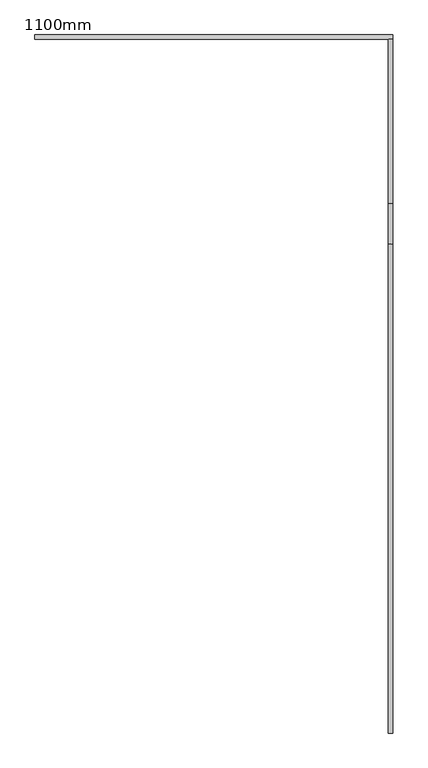
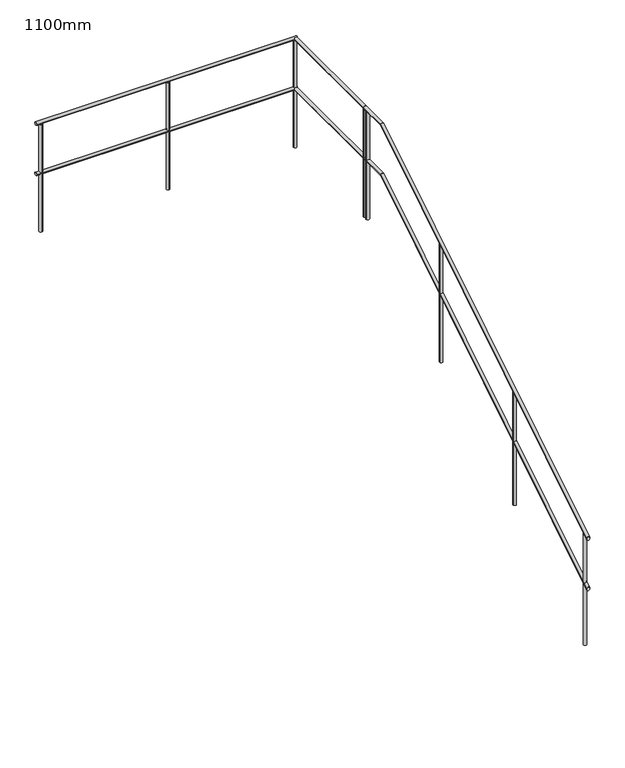
"""IFC4 building model written with IfcOpenShell, lengths in millimetres: railing geometry, 1100mm."""

from ifc_helpers import new_model, si_unit, point, frame, frame_2d, origin, place, context, project, spatial, circle_curve, ellipse_curve, trimmed, segment, composite_curve, outline, extrude, source, transform, mapped, element, save
from ifc_brep_helpers import plane_surface, cylinder_surface, advanced_brep


def railing_1100mm_f57b0715(model_context):
    return source(origin(), model_context, "Body", "SolidModel", [
        advanced_brep(
        [(12685.1052251, 14699.5208589, 456.3396197), (12655.1052251, 14699.5208589, 456.3396197), (12685.1052251, 18339.5208589, 2547.0), (12655.1052251, 18339.5208589, 2547.0), (12685.1052251, 18063.8019306, 2547.0), (12655.1052251, 18063.8019306, 2547.0)],
        [
            (0, 1, ellipse_curve(frame((12670.1052251, 14699.5208589, 456.3396197), z_axis=(0.0, -1.0, 0.0), x_axis=(0.0, 0.0, -1.0)), 17.6603803, 15.0)),
            (1, 0, ellipse_curve(frame((12670.1052251, 14699.5208589, 456.3396197), z_axis=(0.0, -1.0, 0.0), x_axis=(0.0, 0.0, -1.0)), 17.6603803, 15.0)),
            (2, 3, circle_curve(frame((12670.1052251, 18339.5208589, 2547.0), z_axis=(0.0, 1.0, 0.0), x_axis=(-1.0, 0.0, 0.0)), 15.0)),
            (3, 2, circle_curve(frame((12670.1052251, 18339.5208589, 2547.0), z_axis=(0.0, 1.0, 0.0), x_axis=(-1.0, 0.0, 0.0)), 15.0)),
            (0, 4),
            (4, 5, ellipse_curve(frame((12670.1052251, 18063.8019306, 2547.0), z_axis=(0.0, -0.9616025257983003, -0.2744459552959912), x_axis=(0.0, 0.2744459552959914, -0.9616025257983002)), 15.5989607, 15.0)),
            (5, 1),
            (5, 4, ellipse_curve(frame((12670.1052251, 18063.8019306, 2547.0), z_axis=(0.0, -0.9616025257983003, -0.2744459552959912), x_axis=(0.0, 0.2744459552959914, -0.9616025257983002)), 15.5989607, 15.0)),
            (4, 2),
            (3, 5),
        ],
        [
            plane_surface(frame((12670.1052251, 14699.5208589, 474.0), z_axis=(0.0, -1.0, 0.0), x_axis=(0.0, 0.0, 1.0))),
            plane_surface(frame((12670.1052251, 18339.5208589, 2562.0), z_axis=(0.0, 1.0, 0.0), x_axis=(0.0, 0.0, 1.0))),
            cylinder_surface(frame((12670.1052251, 14707.4380966, 461.2596175), z_axis=(0.0, -0.8493588352433417, -0.5278158476155052), x_axis=(-1.0, 0.0, 0.0)), 15.0),
            cylinder_surface(frame((12670.1052251, 18059.5208589, 2547.0), z_axis=(0.0, -1.0, 0.0), x_axis=(-1.0, 0.0, 0.0)), 15.0),
        ],
        [
            (0, [[1, 2]]),
            (1, [[3, 4]]),
            (2, [[-1, 5, 6, 7]]),
            (2, [[-2, -7, 8, -5]]),
            (3, [[-6, 9, -4, 10]]),
            (3, [[-8, -10, -3, -9]]),
        ],
    ),
        advanced_brep(
        [(12685.1052251, 18339.5208589, 2547.0), (12655.1052251, 18339.5208589, 2547.0), (12685.1052251, 19469.5208589, 2547.0), (12655.1052251, 19469.5208589, 2547.0)],
        [
            (0, 1, circle_curve(frame((12670.1052251, 18339.5208589, 2547.0), z_axis=(0.0, -1.0, 0.0), x_axis=(-1.0, 0.0, 0.0)), 15.0)),
            (1, 0, circle_curve(frame((12670.1052251, 18339.5208589, 2547.0), z_axis=(0.0, -1.0, 0.0), x_axis=(-1.0, 0.0, 0.0)), 15.0)),
            (2, 3, circle_curve(frame((12670.1052251, 19469.5208589, 2547.0), z_axis=(0.0, 1.0, 0.0), x_axis=(-1.0, 0.0, 0.0)), 15.0)),
            (3, 2, circle_curve(frame((12670.1052251, 19469.5208589, 2547.0), z_axis=(0.0, 1.0, 0.0), x_axis=(-1.0, 0.0, 0.0)), 15.0)),
            (0, 2),
            (3, 1),
        ],
        [
            plane_surface(frame((12670.1052251, 18339.5208589, 2562.0), z_axis=(0.0, -1.0, 0.0), x_axis=(0.0, 0.0, 1.0))),
            plane_surface(frame((12670.1052251, 19469.5208589, 2562.0), z_axis=(0.0, 1.0, 0.0), x_axis=(0.0, 0.0, 1.0))),
            cylinder_surface(frame((12670.1052251, 18339.5208589, 2547.0), z_axis=(0.0, -1.0, 0.0), x_axis=(-1.0, 0.0, 0.0)), 15.0),
        ],
        [
            (0, [[1, 2]]),
            (1, [[3, 4]]),
            (2, [[-1, 5, -4, 6]]),
            (2, [[-2, -6, -3, -5]]),
        ],
    ),
        advanced_brep(
        [(12685.1052251, 19499.5208589, 2547.0), (12685.1052251, 19469.5208589, 2547.0), (10225.1052251, 19499.5208589, 2547.0), (10225.1052251, 19469.5208589, 2547.0)],
        [
            (0, 1, circle_curve(frame((12685.1052251, 19484.5208589, 2547.0), z_axis=(1.0, 0.0, 0.0), x_axis=(0.0, -1.0, 0.0)), 15.0)),
            (1, 0, circle_curve(frame((12685.1052251, 19484.5208589, 2547.0), z_axis=(1.0, 0.0, 0.0), x_axis=(0.0, -1.0, 0.0)), 15.0)),
            (2, 3, circle_curve(frame((10225.1052251, 19484.5208589, 2547.0), z_axis=(-1.0, 0.0, 0.0), x_axis=(0.0, -1.0, 0.0)), 15.0)),
            (3, 2, circle_curve(frame((10225.1052251, 19484.5208589, 2547.0), z_axis=(-1.0, 0.0, 0.0), x_axis=(0.0, -1.0, 0.0)), 15.0)),
            (0, 2),
            (3, 1),
        ],
        [
            plane_surface(frame((12685.1052251, 19484.5208589, 2562.0), z_axis=(1.0, 0.0, 0.0), x_axis=(0.0, -1.0, 0.0))),
            plane_surface(frame((10225.1052251, 19484.5208589, 2562.0), z_axis=(-1.0, 0.0, 0.0), x_axis=(0.0, -1.0, 0.0))),
            cylinder_surface(frame((12685.1052251, 19484.5208589, 2547.0), z_axis=(1.0, 0.0, 0.0), x_axis=(0.0, -1.0, 0.0)), 15.0),
        ],
        [
            (0, [[1, 2]]),
            (1, [[3, 4]]),
            (2, [[-1, 5, -4, 6]]),
            (2, [[-2, -6, -3, -5]]),
        ],
    ),
        advanced_brep(
        [(12685.1052251, 14699.5208589, 956.3396197), (12655.1052251, 14699.5208589, 956.3396197), (12685.1052251, 18063.8019306, 3047.0), (12655.1052251, 18063.8019306, 3047.0), (12685.1052251, 18339.5208589, 3047.0), (12655.1052251, 18339.5208589, 3047.0)],
        [
            (0, 1, ellipse_curve(frame((12670.1052251, 14699.5208589, 956.3396197), z_axis=(0.0, -1.0, 0.0), x_axis=(0.0, 0.0, -1.0)), 17.6603803, 15.0)),
            (1, 0, ellipse_curve(frame((12670.1052251, 14699.5208589, 956.3396197), z_axis=(0.0, -1.0, 0.0), x_axis=(0.0, 0.0, -1.0)), 17.6603803, 15.0)),
            (0, 2),
            (2, 3, ellipse_curve(frame((12670.1052251, 18063.8019306, 3047.0), z_axis=(0.0, -0.9616025257983003, -0.2744459552959912), x_axis=(0.0, 0.2744459552959914, -0.9616025257983002)), 15.5989607, 15.0)),
            (3, 1),
            (3, 2, ellipse_curve(frame((12670.1052251, 18063.8019306, 3047.0), z_axis=(0.0, -0.9616025257983003, -0.2744459552959912), x_axis=(0.0, 0.2744459552959914, -0.9616025257983002)), 15.5989607, 15.0)),
            (4, 5, circle_curve(frame((12670.1052251, 18339.5208589, 3047.0), z_axis=(0.0, 1.0, 0.0), x_axis=(-1.0, 0.0, 0.0)), 15.0)),
            (5, 4, circle_curve(frame((12670.1052251, 18339.5208589, 3047.0), z_axis=(0.0, 1.0, 0.0), x_axis=(-1.0, 0.0, 0.0)), 15.0)),
            (2, 4),
            (5, 3),
        ],
        [
            plane_surface(frame((12670.1052251, 14699.5208589, 974.0), z_axis=(0.0, -1.0, 0.0), x_axis=(0.0, 0.0, 1.0))),
            cylinder_surface(frame((12670.1052251, 14707.4380966, 961.2596175), z_axis=(0.0, -0.8493588352433417, -0.5278158476155052), x_axis=(-1.0, 0.0, 0.0)), 15.0),
            plane_surface(frame((12670.1052251, 18339.5208589, 3062.0), z_axis=(0.0, 1.0, 0.0), x_axis=(0.0, 0.0, 1.0))),
            cylinder_surface(frame((12670.1052251, 18059.5208589, 3047.0), z_axis=(0.0, -1.0, 0.0), x_axis=(-1.0, 0.0, 0.0)), 15.0),
        ],
        [
            (0, [[1, 2]]),
            (1, [[-1, 3, 4, 5]]),
            (1, [[-2, -5, 6, -3]]),
            (2, [[7, 8]]),
            (3, [[-4, 9, -8, 10]]),
            (3, [[-6, -10, -7, -9]]),
        ],
    ),
        advanced_brep(
        [(12685.1052251, 18339.5208589, 3047.0), (12655.1052251, 18339.5208589, 3047.0), (12685.1052251, 19469.5208589, 3047.0), (12655.1052251, 19469.5208589, 3047.0)],
        [
            (0, 1, circle_curve(frame((12670.1052251, 18339.5208589, 3047.0), z_axis=(0.0, -1.0, 0.0), x_axis=(-1.0, 0.0, 0.0)), 15.0)),
            (1, 0, circle_curve(frame((12670.1052251, 18339.5208589, 3047.0), z_axis=(0.0, -1.0, 0.0), x_axis=(-1.0, 0.0, 0.0)), 15.0)),
            (2, 3, circle_curve(frame((12670.1052251, 19469.5208589, 3047.0), z_axis=(0.0, 1.0, 0.0), x_axis=(-1.0, 0.0, 0.0)), 15.0)),
            (3, 2, circle_curve(frame((12670.1052251, 19469.5208589, 3047.0), z_axis=(0.0, 1.0, 0.0), x_axis=(-1.0, 0.0, 0.0)), 15.0)),
            (0, 2),
            (3, 1),
        ],
        [
            plane_surface(frame((12670.1052251, 18339.5208589, 3062.0), z_axis=(0.0, -1.0, 0.0), x_axis=(0.0, 0.0, 1.0))),
            plane_surface(frame((12670.1052251, 19469.5208589, 3062.0), z_axis=(0.0, 1.0, 0.0), x_axis=(0.0, 0.0, 1.0))),
            cylinder_surface(frame((12670.1052251, 18339.5208589, 3047.0), z_axis=(0.0, -1.0, 0.0), x_axis=(-1.0, 0.0, 0.0)), 15.0),
        ],
        [
            (0, [[1, 2]]),
            (1, [[3, 4]]),
            (2, [[-1, 5, -4, 6]]),
            (2, [[-2, -6, -3, -5]]),
        ],
    ),
        advanced_brep(
        [(12685.1052251, 19499.5208589, 3047.0), (12685.1052251, 19469.5208589, 3047.0), (10225.1052251, 19499.5208589, 3047.0), (10225.1052251, 19469.5208589, 3047.0)],
        [
            (0, 1, circle_curve(frame((12685.1052251, 19484.5208589, 3047.0), z_axis=(1.0, 0.0, 0.0), x_axis=(0.0, -1.0, 0.0)), 15.0)),
            (1, 0, circle_curve(frame((12685.1052251, 19484.5208589, 3047.0), z_axis=(1.0, 0.0, 0.0), x_axis=(0.0, -1.0, 0.0)), 15.0)),
            (2, 3, circle_curve(frame((10225.1052251, 19484.5208589, 3047.0), z_axis=(-1.0, 0.0, 0.0), x_axis=(0.0, -1.0, 0.0)), 15.0)),
            (3, 2, circle_curve(frame((10225.1052251, 19484.5208589, 3047.0), z_axis=(-1.0, 0.0, 0.0), x_axis=(0.0, -1.0, 0.0)), 15.0)),
            (0, 2),
            (3, 1),
        ],
        [
            plane_surface(frame((12685.1052251, 19484.5208589, 3062.0), z_axis=(1.0, 0.0, 0.0), x_axis=(0.0, -1.0, 0.0))),
            plane_surface(frame((10225.1052251, 19484.5208589, 3062.0), z_axis=(-1.0, 0.0, 0.0), x_axis=(0.0, -1.0, 0.0))),
            cylinder_surface(frame((12685.1052251, 19484.5208589, 3047.0), z_axis=(1.0, 0.0, 0.0), x_axis=(0.0, -1.0, 0.0)), 15.0),
        ],
        [
            (0, [[1, 2]]),
            (1, [[3, 4]]),
            (2, [[-1, 5, -4, 6]]),
            (2, [[-2, -6, -3, -5]]),
        ],
    ),
        extrude(outline(composite_curve([segment(trimmed(circle_curve(frame_2d((10270.1052251, 19484.5208589)), 15.0), [point((10270.1052251, 19469.5208589))], [point((10270.1052251, 19499.5208589))], False, "CARTESIAN"), True, "CONTINUOUS"), segment(trimmed(circle_curve(frame_2d((10270.1052251, 19484.5208589)), 15.0), [point((10270.1052251, 19499.5208589))], [point((10270.1052251, 19469.5208589))], False, "CARTESIAN"), True, "CONTINUOUS")], self_intersect=False)), frame((0.0, 0.0, 1962.0), z_axis=(0.0, 0.0, 1.0), x_axis=(1.0, 0.0, 0.0)), (0.0, 0.0, 1.0), 1070.0),
        extrude(outline(composite_curve([segment(trimmed(circle_curve(frame_2d((11470.1052251, 19484.5208589)), 15.0), [point((11470.1052251, 19469.5208589))], [point((11470.1052251, 19499.5208589))], False, "CARTESIAN"), True, "CONTINUOUS"), segment(trimmed(circle_curve(frame_2d((11470.1052251, 19484.5208589)), 15.0), [point((11470.1052251, 19499.5208589))], [point((11470.1052251, 19469.5208589))], False, "CARTESIAN"), True, "CONTINUOUS")], self_intersect=False)), frame((0.0, 0.0, 1962.0), z_axis=(0.0, 0.0, 1.0), x_axis=(1.0, 0.0, 0.0)), (0.0, 0.0, 1.0), 1070.0),
        extrude(outline(composite_curve([segment(trimmed(circle_curve(frame_2d((12670.1052251, 18299.5208589)), 15.0), [point((12655.1052251, 18299.5208589))], [point((12685.1052251, 18299.5208589))], False, "CARTESIAN"), True, "CONTINUOUS"), segment(trimmed(circle_curve(frame_2d((12670.1052251, 18299.5208589)), 15.0), [point((12685.1052251, 18299.5208589))], [point((12655.1052251, 18299.5208589))], False, "CARTESIAN"), True, "CONTINUOUS")], self_intersect=False)), frame((0.0, 0.0, 1962.0), z_axis=(0.0, 0.0, 1.0), x_axis=(1.0, 0.0, 0.0)), (0.0, 0.0, 1.0), 1070.0),
        extrude(outline(composite_curve([segment(trimmed(circle_curve(frame_2d((12670.1052251, 17099.5208589)), 15.0), [point((12655.1052251, 17099.5208589))], [point((12685.1052251, 17099.5208589))], False, "CARTESIAN"), True, "CONTINUOUS"), segment(trimmed(circle_curve(frame_2d((12670.1052251, 17099.5208589)), 15.0), [point((12685.1052251, 17099.5208589))], [point((12655.1052251, 17099.5208589))], False, "CARTESIAN"), True, "CONTINUOUS")], self_intersect=False)), frame((0.0, 0.0, 1266.0), z_axis=(0.0, 0.0, 1.0), x_axis=(1.0, 0.0, 0.0)), (0.0, 0.0, 1.0), 1169.4285714),
        extrude(outline(composite_curve([segment(trimmed(circle_curve(frame_2d((12670.1052251, 15899.5208589)), 15.0), [point((12655.1052251, 15899.5208589))], [point((12685.1052251, 15899.5208589))], False, "CARTESIAN"), True, "CONTINUOUS"), segment(trimmed(circle_curve(frame_2d((12670.1052251, 15899.5208589)), 15.0), [point((12685.1052251, 15899.5208589))], [point((12655.1052251, 15899.5208589))], False, "CARTESIAN"), True, "CONTINUOUS")], self_intersect=False)), frame((0.0, 0.0, 570.0), z_axis=(0.0, 0.0, 1.0), x_axis=(1.0, 0.0, 0.0)), (0.0, 0.0, 1.0), 1119.7142857),
        extrude(outline(composite_curve([segment(trimmed(circle_curve(frame_2d((12670.1052251, 19484.5208589)), 15.0), [point((12655.1052251, 19484.5208589))], [point((12685.1052251, 19484.5208589))], False, "CARTESIAN"), True, "CONTINUOUS"), segment(trimmed(circle_curve(frame_2d((12670.1052251, 19484.5208589)), 15.0), [point((12685.1052251, 19484.5208589))], [point((12655.1052251, 19484.5208589))], False, "CARTESIAN"), True, "CONTINUOUS")], self_intersect=False)), frame((0.0, 0.0, 1962.0), z_axis=(0.0, 0.0, 1.0), x_axis=(1.0, 0.0, 0.0)), (0.0, 0.0, 1.0), 1070.0),
        extrude(outline(composite_curve([segment(trimmed(circle_curve(frame_2d((12670.1052251, 18339.5208589)), 15.0), [point((12655.1052251, 18339.5208589))], [point((12685.1052251, 18339.5208589))], False, "CARTESIAN"), True, "CONTINUOUS"), segment(trimmed(circle_curve(frame_2d((12670.1052251, 18339.5208589)), 15.0), [point((12685.1052251, 18339.5208589))], [point((12655.1052251, 18339.5208589))], False, "CARTESIAN"), True, "CONTINUOUS")], self_intersect=False)), frame((0.0, 0.0, 1962.0), z_axis=(0.0, 0.0, 1.0), x_axis=(1.0, 0.0, 0.0)), (0.0, 0.0, 1.0), 1070.0),
        extrude(outline(composite_curve([segment(trimmed(circle_curve(frame_2d((10275.1052251, 19484.5208589)), 15.0), [point((10275.1052251, 19469.5208589))], [point((10275.1052251, 19499.5208589))], False, "CARTESIAN"), True, "CONTINUOUS"), segment(trimmed(circle_curve(frame_2d((10275.1052251, 19484.5208589)), 15.0), [point((10275.1052251, 19499.5208589))], [point((10275.1052251, 19469.5208589))], False, "CARTESIAN"), True, "CONTINUOUS")], self_intersect=False)), frame((0.0, 0.0, 1962.0), z_axis=(0.0, 0.0, 1.0), x_axis=(1.0, 0.0, 0.0)), (0.0, 0.0, 1.0), 1070.0),
        extrude(outline(composite_curve([segment(trimmed(circle_curve(frame_2d((12670.1052251, 14749.5208589)), 15.0), [point((12655.1052251, 14749.5208589))], [point((12685.1052251, 14749.5208589))], False, "CARTESIAN"), True, "CONTINUOUS"), segment(trimmed(circle_curve(frame_2d((12670.1052251, 14749.5208589)), 15.0), [point((12685.1052251, 14749.5208589))], [point((12655.1052251, 14749.5208589))], False, "CARTESIAN"), True, "CONTINUOUS")], self_intersect=False)), frame((0.0, 0.0, -126.0), z_axis=(0.0, 0.0, 1.0), x_axis=(1.0, 0.0, 0.0)), (0.0, 0.0, 1.0), 1101.0714286),
    ])


if __name__ == "__main__":
    model = new_model("IFC4")
    model_context = context("Model", 3, world=origin())
    ifc_project = project(units=[si_unit("LENGTHUNIT", "METRE", prefix="MILLI")], contexts=[model_context])
    site = spatial("IfcSite", under=ifc_project)
    building = spatial("IfcBuilding", under=site)
    placement = place(None, origin())
    railing_1100mm_shape = railing_1100mm_f57b0715(model_context)
    element("IfcRailing", 1, ObjectType="1100mm", at=placement, inside=building, context=model_context, shape_type="MappedRepresentation", body=[
        mapped(railing_1100mm_shape, transform((0.0, 0.0, 0.0), x_axis=(1.0, 0.0, 0.0), y_axis=(0.0, 1.0, 0.0), z_axis=(0.0, 0.0, 1.0))),
    ])
    save(model, "model.ifc")
